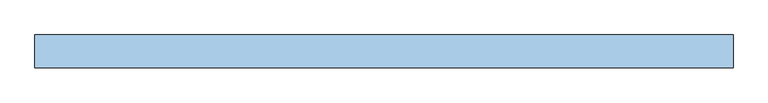
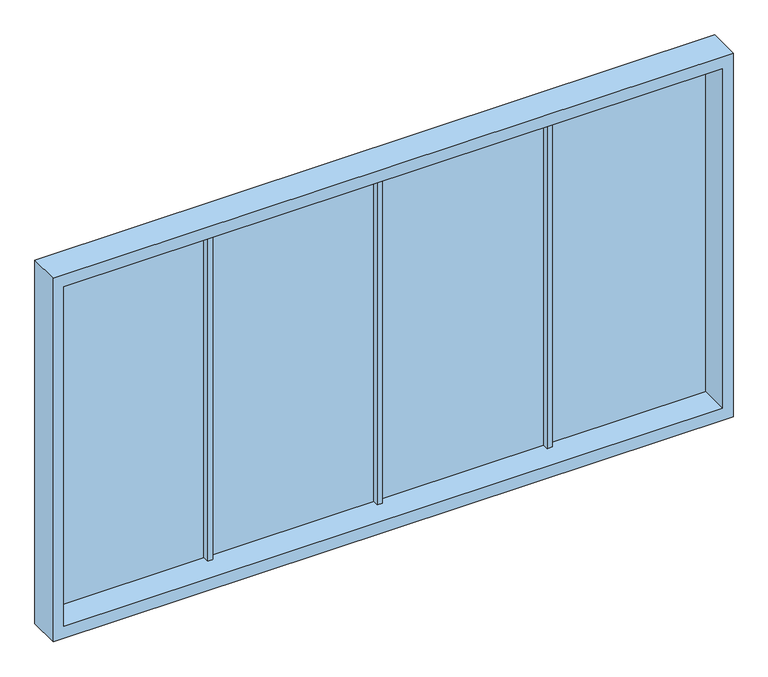
"""IFC4 building model written with IfcOpenShell, lengths in millimetres: window geometry, Finestra Assemblata : vetrata uffici1."""

from ifc_helpers import new_model, si_unit, frame, origin, place, context, project, spatial, polyline, outline, extrude, faceted_brep, source, transform, mapped, element, save


def window_8667a62f(model_context):
    return source(origin(), model_context, "Body", "SolidModel", [
        faceted_brep([(-3255.5, 149.7451428, 3700.0), (3144.5, 149.7451428, 3700.0), (3144.5, 149.7451428, 80.0), (-3255.5, 149.7451428, 80.0), (-3155.5, 149.7451428, 3580.0), (-3155.5, 149.7451428, 200.0), (-1680.2592993, 149.7451428, 200.0), (-1680.2592993, 149.7451428, 3580.0), (-1630.5, 149.7451428, 200.0), (-80.5, 149.7451428, 200.0), (-80.5, 149.7451428, 3580.0), (-1630.5, 149.7451428, 3580.0), (1519.5, 149.7451428, 200.0), (1519.5, 149.7451428, 3580.0), (-30.5, 149.7451428, 3580.0), (-30.5, 149.7451428, 200.0), (1569.5, 149.7451428, 3580.0), (1569.5, 149.7451428, 200.0), (3044.5, 149.7451428, 200.0), (3044.5, 149.7451428, 3580.0), (-3155.5, -150.2548572, 3580.0), (-3155.5, -150.2548572, 200.0), (3044.5, -150.2548572, 200.0), (1569.5, 67.6275467, 200.0), (1519.5, 67.6275467, 200.0), (-30.5, 67.6275467, 200.0), (-80.5, 67.6275467, 200.0), (-1630.5, 67.6275467, 200.0), (-1680.2592993, 67.6275467, 200.0), (-1680.2592993, 67.6275467, 3580.0), (3144.5, -150.2548572, 3700.0), (3144.5, -150.2548572, 80.0), (-3255.5, -150.2548572, 80.0), (-3255.5, -150.2548572, 3700.0), (-80.5, 67.6275467, 3580.0), (-1630.5, 67.6275467, 3580.0), (1519.5, 67.6275467, 3580.0), (-30.5, 67.6275467, 3580.0), (1569.5, 67.6275467, 3580.0), (3044.5, -150.2548572, 3580.0)], [[[0, 1, 2, 3], [4, 5, 6, 7], [8, 9, 10, 11], [12, 13, 14, 15], [16, 17, 18, 19]], [[20, 21, 5, 4]], [[21, 22, 18, 17, 23, 24, 12, 15, 25, 26, 9, 8, 27, 28, 6, 5]], [[7, 6, 28, 29]], [[30, 31, 2, 1]], [[31, 32, 3, 2]], [[32, 33, 0, 3]], [[10, 9, 26, 34]], [[8, 11, 35, 27]], [[13, 12, 24, 36]], [[15, 14, 37, 25]], [[17, 16, 38, 23]], [[22, 39, 19, 18]], [[36, 24, 23, 38]], [[33, 32, 31, 30], [20, 39, 22, 21]], [[34, 26, 25, 37]], [[29, 28, 27, 35]], [[33, 30, 1, 0]], [[39, 20, 4, 7, 29, 35, 11, 10, 34, 37, 14, 13, 36, 38, 16, 19]]]),
        extrude(outline(polyline([(3044.5, 124.7451428), (1569.5, 124.7451428), (1569.5, 134.7451428), (3044.5, 134.7451428), (3044.5, 124.7451428)])), frame((0.0, 0.0, 200.0), z_axis=(0.0, 0.0, 1.0), x_axis=(1.0, 0.0, 0.0)), (0.0, 0.0, 1.0), 3380.0),
        extrude(outline(polyline([(1519.5, 124.7451428), (-30.5, 124.7451428), (-30.5, 134.7451428), (1519.5, 134.7451428), (1519.5, 124.7451428)])), frame((0.0, 0.0, 200.0), z_axis=(0.0, 0.0, 1.0), x_axis=(1.0, 0.0, 0.0)), (0.0, 0.0, 1.0), 3380.0),
        extrude(outline(polyline([(-80.5, 124.7451428), (-1630.5, 124.7451428), (-1630.5, 134.7451428), (-80.5, 134.7451428), (-80.5, 124.7451428)])), frame((0.0, 0.0, 200.0), z_axis=(0.0, 0.0, 1.0), x_axis=(1.0, 0.0, 0.0)), (0.0, 0.0, 1.0), 3380.0),
        extrude(outline(polyline([(-1680.2592993, 124.7451428), (-3155.5, 124.7451428), (-3155.5, 134.7451428), (-1680.2592993, 134.7451428), (-1680.2592993, 124.7451428)])), frame((0.0, 0.0, 200.0), z_axis=(0.0, 0.0, 1.0), x_axis=(1.0, 0.0, 0.0)), (0.0, 0.0, 1.0), 3380.0),
    ])


if __name__ == "__main__":
    model = new_model("IFC4")
    model_context = context("Model", 3, world=origin())
    ifc_project = project(units=[si_unit("LENGTHUNIT", "METRE", prefix="MILLI")], contexts=[model_context])
    site = spatial("IfcSite", under=ifc_project)
    building = spatial("IfcBuilding", under=site)
    placement = place(None, origin())
    window_shape = window_8667a62f(model_context)
    element("IfcWindow", 1, ObjectType="Finestra Assemblata : vetrata uffici1", at=placement, inside=building, context=model_context, shape_type="MappedRepresentation", body=[
        mapped(window_shape, transform((0.0, 0.0, 0.0), x_axis=(1.0, 0.0, 0.0), y_axis=(0.0, 1.0, 0.0), z_axis=(0.0, 0.0, 1.0))),
    ])
    save(model, "model.ifc")

# Revit data of these elements
# Type "Finestra Assemblata : vetrata uffici1"
#   Type Mark = "33"
#   Construction Type Id = "GSP4R"
#   Analytic Construction = "Vetrata singola Pilkington 1/8 in"
#   Visual Light Transmittance = 0.9
#   Solar Heat Gain Coefficient = 0.78
#   Heat Transfer Coefficient (U) = 3.6886 W/(m²·K)
#   MONTANTE = 1.60 m
#   Luce sup = 0.50 m
#   Height = 3.60 m
#   Altezza soglia = 0.10 m
#   Width = 6.40 m
#   Vetro = Default - Vetro
#   Telaio/montante = Metallo - Acciaio inox, levigato
#   Davanzale = Metallo - Acciaio inox, levigato
#   Manufacturer = ""
#   Wall Closure = (empty or 0)
# Element 1 (IfcWindow, "Finestra Assemblata : vetrata uffici1")
#   Materials on its faces: "Metallo - Acciaio inox, levigato", "Default - Vetro"
# Materials
#   "Default - Vetro": class "Vetro", colour RGB 208 208 208, transparency 0.7, Cost = 0
#   "Metallo - Acciaio inox, levigato": class "Metallo", colour RGB 236 239 239, transparency 0, Cost = 0
